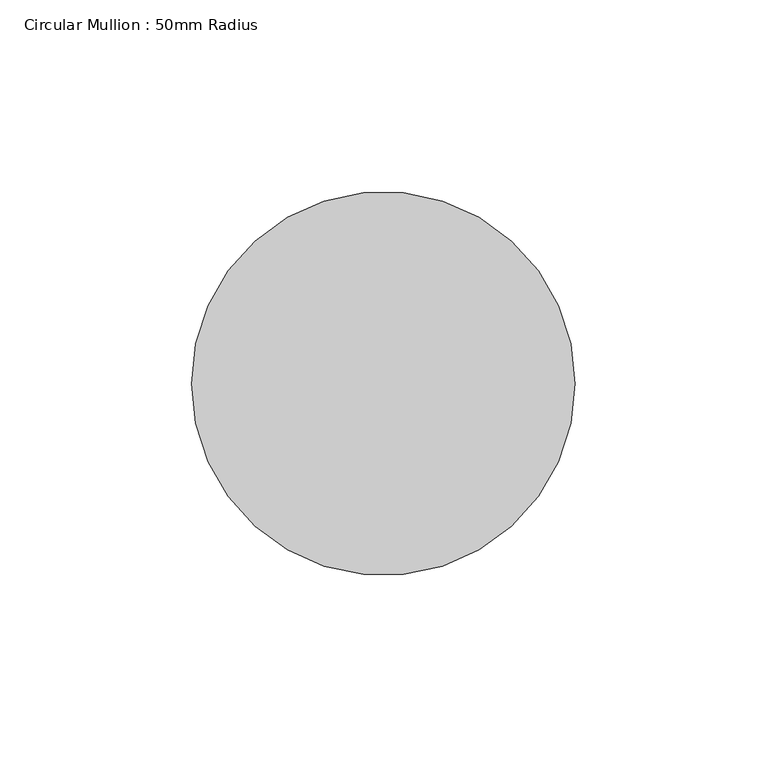
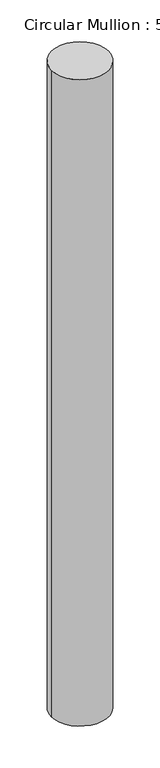
"""IFC4 building model written with IfcOpenShell, lengths in millimetres: member geometry, Circular Mullion : 50mm Radius."""

from ifc_helpers import new_model, si_unit, point, frame, origin, origin_2d, place, context, project, spatial, circle_curve, trimmed, segment, composite_curve, outline, extrude, source, transform, mapped, element, save


def circular_mullion_50mm_radius_eec866e4(model_context):
    return source(origin(), model_context, "Body", "SweptSolid", [
        extrude(outline(composite_curve([segment(trimmed(circle_curve(origin_2d(), 50.0), [point((50.0, 0.0))], [point((-50.0, 0.0))], False, "CARTESIAN"), True, "CONTINUOUS"), segment(trimmed(circle_curve(origin_2d(), 50.0), [point((-50.0, 0.0))], [point((50.0, 0.0))], False, "CARTESIAN"), True, "CONTINUOUS")], self_intersect=False)), frame((0.0, 0.0, -1195.4728618), z_axis=(0.0, 0.0, 1.0), x_axis=(1.0, 0.0, 0.0)), (0.0, 0.0, 1.0), 1195.4728618),
    ])


if __name__ == "__main__":
    model = new_model("IFC4")
    model_context = context("Model", 3, world=origin())
    ifc_project = project(units=[si_unit("LENGTHUNIT", "METRE", prefix="MILLI")], contexts=[model_context])
    site = spatial("IfcSite", under=ifc_project)
    building = spatial("IfcBuilding", under=site)
    placement = place(None, origin())
    circular_mullion_50mm_radius_shape = circular_mullion_50mm_radius_eec866e4(model_context)
    element("IfcMember", 1, ObjectType="Circular Mullion : 50mm Radius", at=placement, inside=building, context=model_context, shape_type="MappedRepresentation", body=[
        mapped(circular_mullion_50mm_radius_shape, transform((0.0, 0.0, 0.0), x_axis=(1.0, 0.0, 0.0), y_axis=(0.0, 1.0, 0.0), z_axis=(0.0, 0.0, 1.0))),
    ])
    save(model, "model.ifc")

# Revit data of these elements
# Type "Circular Mullion : 50mm Radius"
#   built-in parameter 1007350 = 0.164042 (stored number, unit not read)
# Element 1 (IfcMember, "Circular Mullion : 50mm Radius")
#   Materials on its faces: "Aluminium"
# Materials
#   "Aluminium": class "Metal", colour RGB 247 247 247, transparency 0, Description = "Aluminium 6061", Cost = 0
